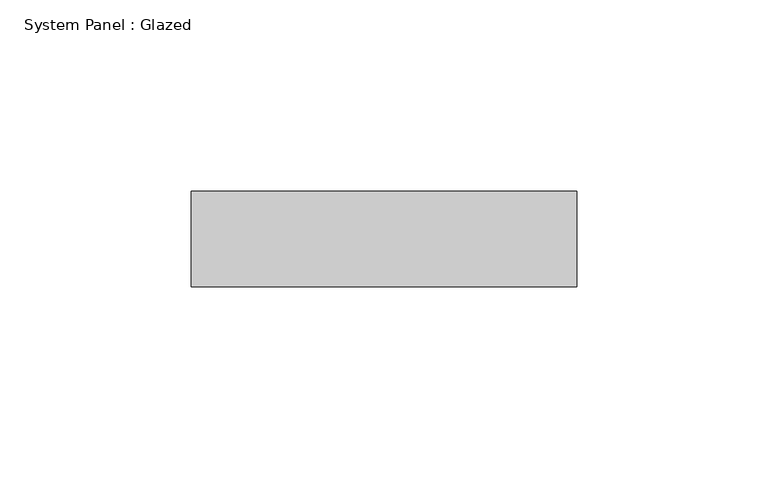
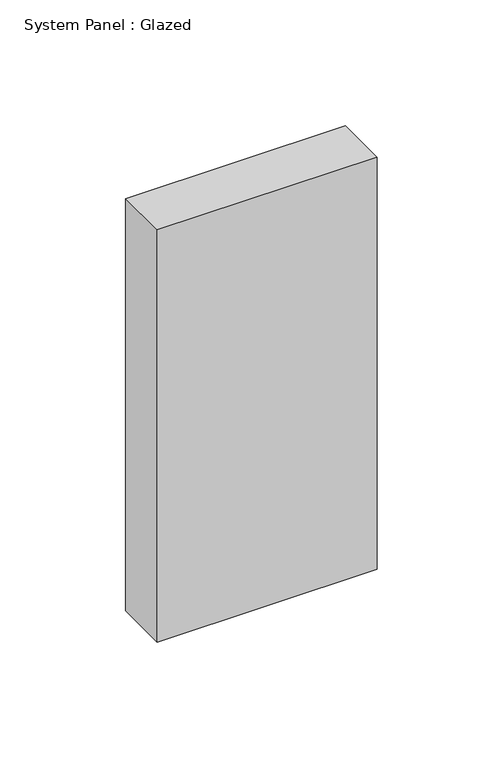
"""IFC4 building model written with IfcOpenShell, lengths in millimetres: plate geometry, System Panel : Glazed."""

from ifc_helpers import new_model, si_unit, origin, origin_with_axes, place, context, project, spatial, polyline, outline, extrude, source, transform, mapped, element, save


def system_panel_glazed_b9ee7cbb(model_context):
    return source(origin(), model_context, "Body", "SweptSolid", [
        extrude(outline(polyline([(50.5028251, 24.5), (-50.5028251, 24.5), (-50.5028251, 49.5), (50.5028251, 49.5), (50.5028251, 24.5)])), origin_with_axes(), (0.0, 0.0, 1.0), 200.0),
    ])


if __name__ == "__main__":
    model = new_model("IFC4")
    model_context = context("Model", 3, world=origin())
    ifc_project = project(units=[si_unit("LENGTHUNIT", "METRE", prefix="MILLI")], contexts=[model_context])
    site = spatial("IfcSite", under=ifc_project)
    building = spatial("IfcBuilding", under=site)
    placement = place(None, origin())
    system_panel_glazed_shape = system_panel_glazed_b9ee7cbb(model_context)
    element("IfcPlate", 1, ObjectType="System Panel : Glazed", at=placement, inside=building, context=model_context, shape_type="MappedRepresentation", body=[
        mapped(system_panel_glazed_shape, transform((0.0, 0.0, 0.0), x_axis=(1.0, 0.0, 0.0), y_axis=(0.0, 1.0, 0.0), z_axis=(0.0, 0.0, 1.0))),
    ])
    save(model, "model.ifc")

# Revit data of these elements
# Element 1 (IfcPlate, "System Panel : Glazed")
#   Materials on its faces: "Glass"
# Materials
#   "Glass": class "Glass", colour RGB 218 227 224, transparency 0.85, Description = "Soda Lime Glass", Cost = 0
